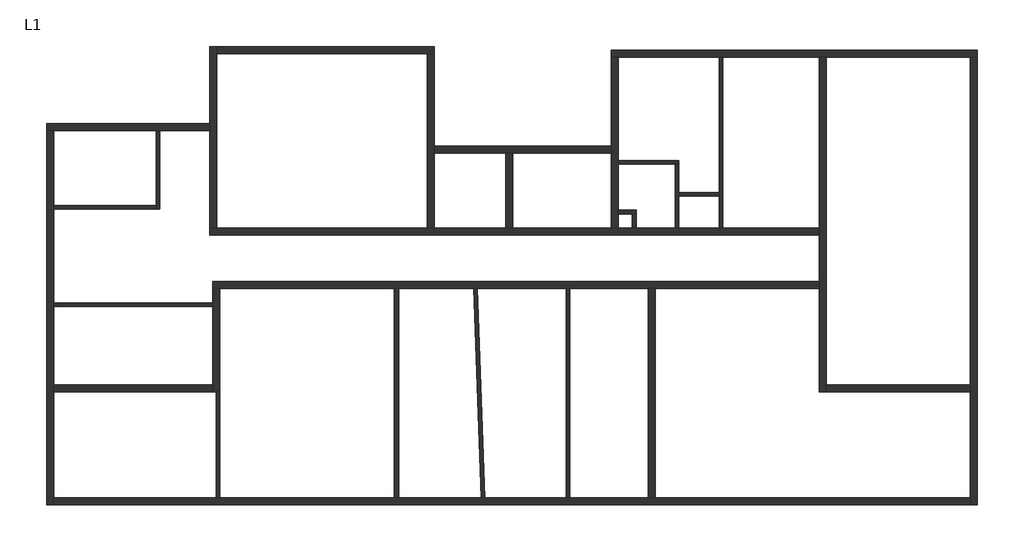
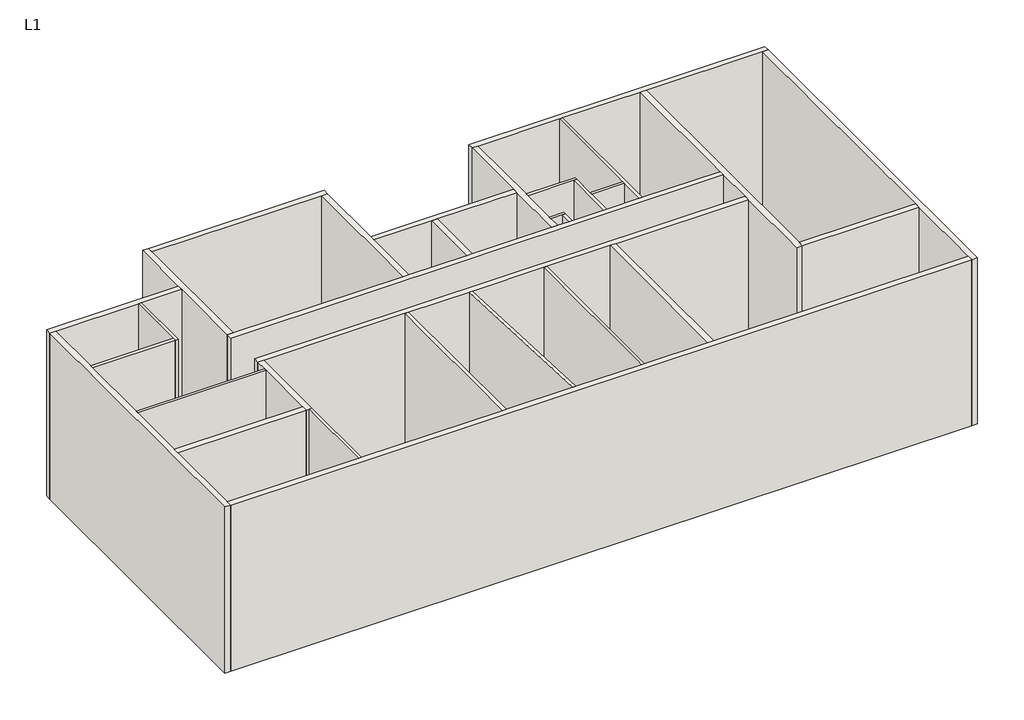
# One storey: 31 walls.
"""IFC4 building model written with IfcOpenShell, lengths in millimetres."""

from ifc_helpers import new_model, si_unit, origin, origin_with_axes, place, context, project, spatial, polyline, outline, extrude, faceted_brep, element, save

model = new_model("IFC4")

# Units and contexts
model_context = context("Model", 3, world=origin())
ifc_project = project(units=[si_unit("LENGTHUNIT", "METRE", prefix="MILLI")], contexts=[model_context])

# Site, building, storey
site = spatial("IfcSite", under=ifc_project)
building = spatial("IfcBuilding", under=site)
storey = spatial("IfcBuildingStorey", under=building, Name="L1", Elevation=0.0)

# Walls
placement = place(None, origin())
element("IfcWall", 1, ObjectType="Generic - 100mm", at=placement, inside=storey, context=model_context, shape_type="Brep", body=[
    faceted_brep([(-11422.4352558, 5591.031319, 0.0), (-11422.4352558, 3491.031319, 0.0), (-11422.4352558, 3391.031319, 0.0), (-11422.4352558, 3391.031319, 6096.0), (-11422.4352558, 3491.031319, 6096.0), (-11422.4352558, 5591.031319, 6096.0), (-11322.4352558, 5591.031319, 0.0), (-11322.4352558, 5591.031319, 6096.0), (-11322.4352558, 3391.031319, 6096.0), (-11322.4352558, 3391.031319, 0.0)], [[[0, 1, 2, 3, 4, 5]], [[6, 7, 8, 9]], [[2, 1, 0, 6, 9]], [[5, 4, 3, 8, 7]], [[0, 5, 7, 6]], [[3, 2, 9, 8]]]),
])
element("IfcWall", 2, ObjectType="Generic - 100mm", at=placement, inside=storey, context=model_context, shape_type="SweptSolid", body=[
    extrude(outline(polyline([(-14299.9378813, 3491.031319), (-11422.4352558, 3491.031319), (-11422.4352558, 3391.031319), (-14299.9378813, 3391.031319), (-14299.9378813, 3491.031319)])), origin_with_axes(), (0.0, 0.0, 1.0), 6096.0),
])
element("IfcWall", 3, ObjectType="Generic - 100mm", at=placement, inside=storey, context=model_context, shape_type="SweptSolid", body=[
    extrude(outline(polyline([(-9843.4352558, 651.031319), (-14299.9378813, 651.031319), (-14299.9378813, 751.031319), (-9843.4352558, 751.031319), (-9843.4352558, 651.031319)])), origin_with_axes(), (0.0, 0.0, 1.0), 6096.0),
])
element("IfcWall", 4, ObjectType="Generic - 100mm", at=placement, inside=storey, context=model_context, shape_type="SweptSolid", body=[
    extrude(outline(polyline([(-9643.4352558, -1748.968681), (-9643.4352558, -4724.7581907), (-9743.4352558, -4724.7581907), (-9743.4352558, -1748.968681), (-9643.4352558, -1748.968681)])), origin_with_axes(), (0.0, 0.0, 1.0), 6096.0),
])
element("IfcWall", 5, ObjectType="Generic - 100mm", at=placement, inside=storey, context=model_context, shape_type="SweptSolid", body=[
    extrude(outline(polyline([(-2303.3408114, -4724.7581907), (-2508.5279024, 1151.031319), (-2408.466948, 1151.031319), (-2203.2798569, -4724.7581907), (-2303.3408114, -4724.7581907)])), origin_with_axes(), (0.0, 0.0, 1.0), 6096.0),
])
element("IfcWall", 6, ObjectType="Generic - 100mm", at=placement, inside=storey, context=model_context, shape_type="SweptSolid", body=[
    extrude(outline(polyline([(77.5647442, -4724.7581907), (77.5647442, 1151.031319), (177.5647442, 1151.031319), (177.5647442, -4724.7581907), (77.5647442, -4724.7581907)])), origin_with_axes(), (0.0, 0.0, 1.0), 6096.0),
])
element("IfcWall", 7, ObjectType="Generic - 100mm", at=placement, inside=storey, context=model_context, shape_type="Brep", body=[
    faceted_brep([(4377.5647442, 7651.031319, 0.0), (4377.5647442, 3851.031319, 0.0), (4377.5647442, 3751.031319, 0.0), (4377.5647442, 2851.031319, 0.0), (4377.5647442, 2851.031319, 6096.0), (4377.5647442, 3751.031319, 6096.0), (4377.5647442, 3851.031319, 6096.0), (4377.5647442, 7651.031319, 6096.0), (4477.5647442, 7651.031319, 0.0), (4477.5647442, 7651.031319, 6096.0), (4477.5647442, 2851.031319, 6096.0), (4477.5647442, 2851.031319, 0.0)], [[[0, 1, 2, 3, 4, 5, 6, 7]], [[8, 9, 10, 11]], [[3, 2, 1, 0, 8, 11]], [[7, 6, 5, 4, 10, 9]], [[0, 7, 9, 8]], [[4, 3, 11, 10]]]),
])
element("IfcWall", 8, ObjectType="Generic - 100mm", at=placement, inside=storey, context=model_context, shape_type="Brep", body=[
    faceted_brep([(1538.9703153, 4651.031319, 0.0), (3138.9703153, 4651.031319, 0.0), (3238.9703153, 4651.031319, 0.0), (3238.9703153, 4651.031319, 6096.0), (3138.9703153, 4651.031319, 6096.0), (1538.9703153, 4651.031319, 6096.0), (1538.9703153, 4751.031319, 0.0), (1538.9703153, 4751.031319, 6096.0), (3238.9703153, 4751.031319, 6096.0), (3238.9703153, 4751.031319, 0.0)], [[[0, 1, 2, 3, 4, 5]], [[6, 7, 8, 9]], [[2, 1, 0, 6, 9]], [[5, 4, 3, 8, 7]], [[0, 5, 7, 6]], [[3, 2, 9, 8]]]),
])
element("IfcWall", 9, ObjectType="Generic - 100mm", at=placement, inside=storey, context=model_context, shape_type="Brep", body=[
    faceted_brep([(3138.9703153, 4651.031319, 0.0), (3138.9703153, 2851.031319, 0.0), (3138.9703153, 2851.031319, 6096.0), (3138.9703153, 4651.031319, 6096.0), (3238.9703153, 4651.031319, 0.0), (3238.9703153, 4651.031319, 6096.0), (3238.9703153, 3851.031319, 6096.0), (3238.9703153, 3751.031319, 6096.0), (3238.9703153, 2851.031319, 6096.0), (3238.9703153, 2851.031319, 0.0), (3238.9703153, 3751.031319, 0.0), (3238.9703153, 3851.031319, 0.0)], [[[0, 1, 2, 3]], [[4, 5, 6, 7, 8, 9, 10, 11]], [[1, 0, 4, 11, 10, 9]], [[3, 2, 8, 7, 6, 5]], [[0, 3, 5, 4]], [[2, 1, 9, 8]]]),
])
element("IfcWall", 10, ObjectType="Generic - 100mm", at=placement, inside=storey, context=model_context, shape_type="Brep", body=[
    faceted_brep([(1538.9703153, 3251.031319, 0.0), (1938.9703153, 3251.031319, 0.0), (2038.9703153, 3251.031319, 0.0), (2038.9703153, 3251.031319, 6096.0), (1938.9703153, 3251.031319, 6096.0), (1538.9703153, 3251.031319, 6096.0), (1538.9703153, 3351.031319, 0.0), (1538.9703153, 3351.031319, 6096.0), (2038.9703153, 3351.031319, 6096.0), (2038.9703153, 3351.031319, 0.0)], [[[0, 1, 2, 3, 4, 5]], [[6, 7, 8, 9]], [[2, 1, 0, 6, 9]], [[5, 4, 3, 8, 7]], [[0, 5, 7, 6]], [[3, 2, 9, 8]]]),
])
element("IfcWall", 11, ObjectType="Generic - 100mm", at=placement, inside=storey, context=model_context, shape_type="SweptSolid", body=[
    extrude(outline(polyline([(1938.9703153, 2851.031319), (1938.9703153, 3251.031319), (2038.9703153, 3251.031319), (2038.9703153, 2851.031319), (1938.9703153, 2851.031319)])), origin_with_axes(), (0.0, 0.0, 1.0), 6096.0),
])
element("IfcWall", 12, ObjectType="Generic - 100mm", at=placement, inside=storey, context=model_context, shape_type="SweptSolid", body=[
    extrude(outline(polyline([(4377.5647442, 3751.031319), (3238.9703153, 3751.031319), (3238.9703153, 3851.031319), (4377.5647442, 3851.031319), (4377.5647442, 3751.031319)])), origin_with_axes(), (0.0, 0.0, 1.0), 6096.0),
])
element("IfcWall", 13, ObjectType="Generic - 200mm", at=placement, inside=storey, context=model_context, shape_type="Brep", body=[
    faceted_brep([(11419.092187, 7651.031319, 0.0), (11419.092187, -1548.968681, 0.0), (11419.092187, -1748.968681, 0.0), (11419.092187, -4724.7581907, 0.0), (11419.092187, -4924.7581907, 0.0), (11419.092187, -4924.7581907, 6096.0), (11419.092187, -4724.7581907, 6096.0), (11419.092187, -1748.968681, 6096.0), (11419.092187, -1548.968681, 6096.0), (11419.092187, 7651.031319, 6096.0), (11619.092187, 7651.031319, 0.0), (11619.092187, 7651.031319, 6096.0), (11619.092187, -4924.7581907, 6096.0), (11619.092187, -4924.7581907, 0.0)], [[[0, 1, 2, 3, 4, 5, 6, 7, 8, 9]], [[10, 11, 12, 13]], [[4, 3, 2, 1, 0, 10, 13]], [[9, 8, 7, 6, 5, 12, 11]], [[5, 4, 13, 12]], [[0, 9, 11, 10]]]),
])
element("IfcWall", 14, ObjectType="Generic - 200mm", at=placement, inside=storey, context=model_context, shape_type="Brep", body=[
    faceted_brep([(11419.092187, -4724.7581907, 0.0), (2577.5647442, -4724.7581907, 0.0), (2377.5647442, -4724.7581907, 0.0), (177.5647442, -4724.7581907, 0.0), (77.5647442, -4724.7581907, 0.0), (-2203.2798569, -4724.7581907, 0.0), (-2303.3408114, -4724.7581907, 0.0), (-4622.4352558, -4724.7581907, 0.0), (-4743.4352558, -4724.7581907, 0.0), (-9643.4352558, -4724.7581907, 0.0), (-9743.4352558, -4724.7581907, 0.0), (-14299.9378813, -4724.7581907, 0.0), (-14299.9378813, -4724.7581907, 6096.0), (-9743.4352558, -4724.7581907, 6096.0), (-9643.4352558, -4724.7581907, 6096.0), (-4743.4352558, -4724.7581907, 6096.0), (-4622.4352558, -4724.7581907, 6096.0), (-2303.3408114, -4724.7581907, 6096.0), (-2203.2798569, -4724.7581907, 6096.0), (77.5647442, -4724.7581907, 6096.0), (177.5647442, -4724.7581907, 6096.0), (2377.5647442, -4724.7581907, 6096.0), (2577.5647442, -4724.7581907, 6096.0), (11419.092187, -4724.7581907, 6096.0), (11419.092187, -4924.7581907, 0.0), (11419.092187, -4924.7581907, 6096.0), (-14299.9378813, -4924.7581907, 6096.0), (-14299.9378813, -4924.7581907, 0.0)], [[[0, 1, 2, 3, 4, 5, 6, 7, 8, 9, 10, 11, 12, 13, 14, 15, 16, 17, 18, 19, 20, 21, 22, 23]], [[24, 25, 26, 27]], [[11, 10, 9, 8, 7, 6, 5, 4, 3, 2, 1, 0, 24, 27]], [[23, 22, 21, 20, 19, 18, 17, 16, 15, 14, 13, 12, 26, 25]], [[0, 23, 25, 24]], [[12, 11, 27, 26]]]),
])
element("IfcWall", 15, ObjectType="Generic - 200mm", at=placement, inside=storey, context=model_context, shape_type="Brep", body=[
    faceted_brep([(-14299.9378813, -4924.7581907, 0.0), (-14299.9378813, -4724.7581907, 0.0), (-14299.9378813, -1748.968681, 0.0), (-14299.9378813, -1548.968681, 0.0), (-14299.9378813, 651.031319, 0.0), (-14299.9378813, 751.031319, 0.0), (-14299.9378813, 3391.031319, 0.0), (-14299.9378813, 3491.031319, 0.0), (-14299.9378813, 5591.031319, 0.0), (-14299.9378813, 5591.031319, 6096.0), (-14299.9378813, 3491.031319, 6096.0), (-14299.9378813, 3391.031319, 6096.0), (-14299.9378813, 751.031319, 6096.0), (-14299.9378813, 651.031319, 6096.0), (-14299.9378813, -1548.968681, 6096.0), (-14299.9378813, -1748.968681, 6096.0), (-14299.9378813, -4724.7581907, 6096.0), (-14299.9378813, -4924.7581907, 6096.0), (-14499.9378813, -4924.7581907, 0.0), (-14499.9378813, -4924.7581907, 6096.0), (-14499.9378813, 5591.031319, 6096.0), (-14499.9378813, 5591.031319, 0.0)], [[[0, 1, 2, 3, 4, 5, 6, 7, 8, 9, 10, 11, 12, 13, 14, 15, 16, 17]], [[18, 19, 20, 21]], [[8, 7, 6, 5, 4, 3, 2, 1, 0, 18, 21]], [[17, 16, 15, 14, 13, 12, 11, 10, 9, 20, 19]], [[9, 8, 21, 20]], [[0, 17, 19, 18]]]),
])
element("IfcWall", 16, ObjectType="Generic - 200mm", at=placement, inside=storey, context=model_context, shape_type="Brep", body=[
    faceted_brep([(-14499.9378813, 5591.031319, 0.0), (-14299.9378813, 5591.031319, 0.0), (-11422.4352558, 5591.031319, 0.0), (-11322.4352558, 5591.031319, 0.0), (-9922.4352558, 5591.031319, 0.0), (-9922.4352558, 5591.031319, 6096.0), (-11322.4352558, 5591.031319, 6096.0), (-11422.4352558, 5591.031319, 6096.0), (-14299.9378813, 5591.031319, 6096.0), (-14499.9378813, 5591.031319, 6096.0), (-14499.9378813, 5791.031319, 0.0), (-14499.9378813, 5791.031319, 6096.0), (-9922.4352558, 5791.031319, 6096.0), (-9922.4352558, 5791.031319, 0.0)], [[[0, 1, 2, 3, 4, 5, 6, 7, 8, 9]], [[10, 11, 12, 13]], [[4, 3, 2, 1, 0, 10, 13]], [[9, 8, 7, 6, 5, 12, 11]], [[5, 4, 13, 12]], [[0, 9, 11, 10]]]),
])
element("IfcWall", 17, ObjectType="Generic - 200mm", at=placement, inside=storey, context=model_context, shape_type="Brep", body=[
    faceted_brep([(-9722.4352558, 2851.031319, 0.0), (-9722.4352558, 7751.031319, 0.0), (-9722.4352558, 7951.031319, 0.0), (-9722.4352558, 7951.031319, 6096.0), (-9722.4352558, 7751.031319, 6096.0), (-9722.4352558, 2851.031319, 6096.0), (-9922.4352558, 2851.031319, 0.0), (-9922.4352558, 2851.031319, 6096.0), (-9922.4352558, 5591.031319, 6096.0), (-9922.4352558, 5791.031319, 6096.0), (-9922.4352558, 7951.031319, 6096.0), (-9922.4352558, 7951.031319, 0.0), (-9922.4352558, 5791.031319, 0.0), (-9922.4352558, 5591.031319, 0.0)], [[[0, 1, 2, 3, 4, 5]], [[6, 7, 8, 9, 10, 11, 12, 13]], [[2, 1, 0, 6, 13, 12, 11]], [[5, 4, 3, 10, 9, 8, 7]], [[3, 2, 11, 10]], [[0, 5, 7, 6]]]),
])
element("IfcWall", 18, ObjectType="Generic - 200mm", at=placement, inside=storey, context=model_context, shape_type="Brep", body=[
    faceted_brep([(-9722.4352558, 7751.031319, 0.0), (-3822.4352558, 7751.031319, 0.0), (-3622.4352558, 7751.031319, 0.0), (-3622.4352558, 7751.031319, 6096.0), (-3822.4352558, 7751.031319, 6096.0), (-9722.4352558, 7751.031319, 6096.0), (-9722.4352558, 7951.031319, 0.0), (-9722.4352558, 7951.031319, 6096.0), (-3622.4352558, 7951.031319, 6096.0), (-3622.4352558, 7951.031319, 0.0)], [[[0, 1, 2, 3, 4, 5]], [[6, 7, 8, 9]], [[2, 1, 0, 6, 9]], [[5, 4, 3, 8, 7]], [[0, 5, 7, 6]], [[3, 2, 9, 8]]]),
])
element("IfcWall", 19, ObjectType="Generic - 200mm", at=placement, inside=storey, context=model_context, shape_type="Brep", body=[
    faceted_brep([(-3822.4352558, 7751.031319, 0.0), (-3822.4352558, 2851.031319, 0.0), (-3822.4352558, 2851.031319, 6096.0), (-3822.4352558, 7751.031319, 6096.0), (-3622.4352558, 7751.031319, 0.0), (-3622.4352558, 7751.031319, 6096.0), (-3622.4352558, 5151.031319, 6096.0), (-3622.4352558, 4951.031319, 6096.0), (-3622.4352558, 2851.031319, 6096.0), (-3622.4352558, 2851.031319, 0.0), (-3622.4352558, 4951.031319, 0.0), (-3622.4352558, 5151.031319, 0.0)], [[[0, 1, 2, 3]], [[4, 5, 6, 7, 8, 9, 10, 11]], [[1, 0, 4, 11, 10, 9]], [[3, 2, 8, 7, 6, 5]], [[0, 3, 5, 4]], [[2, 1, 9, 8]]]),
])
element("IfcWall", 20, ObjectType="Generic - 200mm", at=placement, inside=storey, context=model_context, shape_type="Brep", body=[
    faceted_brep([(-3622.4352558, 4951.031319, 0.0), (-1622.4352558, 4951.031319, 0.0), (-1422.4352558, 4951.031319, 0.0), (1338.9703153, 4951.031319, 0.0), (1338.9703153, 4951.031319, 6096.0), (-1422.4352558, 4951.031319, 6096.0), (-1622.4352558, 4951.031319, 6096.0), (-3622.4352558, 4951.031319, 6096.0), (-3622.4352558, 5151.031319, 0.0), (-3622.4352558, 5151.031319, 6096.0), (1338.9703153, 5151.031319, 6096.0), (1338.9703153, 5151.031319, 0.0)], [[[0, 1, 2, 3, 4, 5, 6, 7]], [[8, 9, 10, 11]], [[3, 2, 1, 0, 8, 11]], [[7, 6, 5, 4, 10, 9]], [[0, 7, 9, 8]], [[4, 3, 11, 10]]]),
])
element("IfcWall", 21, ObjectType="Generic - 200mm", at=placement, inside=storey, context=model_context, shape_type="Brep", body=[
    faceted_brep([(1338.9703153, 7651.031319, 0.0), (1538.9703153, 7651.031319, 0.0), (4377.5647442, 7651.031319, 0.0), (4477.5647442, 7651.031319, 0.0), (7177.5647442, 7651.031319, 0.0), (7377.5647442, 7651.031319, 0.0), (11419.092187, 7651.031319, 0.0), (11619.092187, 7651.031319, 0.0), (11619.092187, 7651.031319, 6096.0), (11419.092187, 7651.031319, 6096.0), (7377.5647442, 7651.031319, 6096.0), (7177.5647442, 7651.031319, 6096.0), (4477.5647442, 7651.031319, 6096.0), (4377.5647442, 7651.031319, 6096.0), (1538.9703153, 7651.031319, 6096.0), (1338.9703153, 7651.031319, 6096.0), (1338.9703153, 7851.031319, 0.0), (1338.9703153, 7851.031319, 6096.0), (11619.092187, 7851.031319, 6096.0), (11619.092187, 7851.031319, 0.0)], [[[0, 1, 2, 3, 4, 5, 6, 7, 8, 9, 10, 11, 12, 13, 14, 15]], [[16, 17, 18, 19]], [[7, 6, 5, 4, 3, 2, 1, 0, 16, 19]], [[15, 14, 13, 12, 11, 10, 9, 8, 18, 17]], [[8, 7, 19, 18]], [[0, 15, 17, 16]]]),
])
element("IfcWall", 22, ObjectType="Generic - 200mm", at=placement, inside=storey, context=model_context, shape_type="Brep", body=[
    faceted_brep([(7177.5647442, 7651.031319, 0.0), (7177.5647442, 2851.031319, 0.0), (7177.5647442, 2651.031319, 0.0), (7177.5647442, 1351.031319, 0.0), (7177.5647442, 1151.031319, 0.0), (7177.5647442, -1748.968681, 0.0), (7177.5647442, -1748.968681, 6096.0), (7177.5647442, 1151.031319, 6096.0), (7177.5647442, 1351.031319, 6096.0), (7177.5647442, 2651.031319, 6096.0), (7177.5647442, 2851.031319, 6096.0), (7177.5647442, 7651.031319, 6096.0), (7377.5647442, 7651.031319, 0.0), (7377.5647442, 7651.031319, 6096.0), (7377.5647442, -1548.968681, 6096.0), (7377.5647442, -1748.968681, 6096.0), (7377.5647442, -1748.968681, 0.0), (7377.5647442, -1548.968681, 0.0)], [[[0, 1, 2, 3, 4, 5, 6, 7, 8, 9, 10, 11]], [[12, 13, 14, 15, 16, 17]], [[5, 4, 3, 2, 1, 0, 12, 17, 16]], [[11, 10, 9, 8, 7, 6, 15, 14, 13]], [[0, 11, 13, 12]], [[6, 5, 16, 15]]]),
])
element("IfcWall", 23, ObjectType="Generic - 200mm", at=placement, inside=storey, context=model_context, shape_type="Brep", body=[
    faceted_brep([(7177.5647442, 2851.031319, 0.0), (4477.5647442, 2851.031319, 0.0), (4377.5647442, 2851.031319, 0.0), (3238.9703153, 2851.031319, 0.0), (3138.9703153, 2851.031319, 0.0), (2038.9703153, 2851.031319, 0.0), (1938.9703153, 2851.031319, 0.0), (1538.9703153, 2851.031319, 0.0), (1338.9703153, 2851.031319, 0.0), (-1422.4352558, 2851.031319, 0.0), (-1622.4352558, 2851.031319, 0.0), (-3622.4352558, 2851.031319, 0.0), (-3822.4352558, 2851.031319, 0.0), (-9722.4352558, 2851.031319, 0.0), (-9922.4352558, 2851.031319, 0.0), (-9922.4352558, 2851.031319, 6096.0), (-9722.4352558, 2851.031319, 6096.0), (-3822.4352558, 2851.031319, 6096.0), (-3622.4352558, 2851.031319, 6096.0), (-1622.4352558, 2851.031319, 6096.0), (-1422.4352558, 2851.031319, 6096.0), (1338.9703153, 2851.031319, 6096.0), (1538.9703153, 2851.031319, 6096.0), (1938.9703153, 2851.031319, 6096.0), (2038.9703153, 2851.031319, 6096.0), (3138.9703153, 2851.031319, 6096.0), (3238.9703153, 2851.031319, 6096.0), (4377.5647442, 2851.031319, 6096.0), (4477.5647442, 2851.031319, 6096.0), (7177.5647442, 2851.031319, 6096.0), (7177.5647442, 2651.031319, 0.0), (7177.5647442, 2651.031319, 6096.0), (-9922.4352558, 2651.031319, 6096.0), (-9922.4352558, 2651.031319, 0.0)], [[[0, 1, 2, 3, 4, 5, 6, 7, 8, 9, 10, 11, 12, 13, 14, 15, 16, 17, 18, 19, 20, 21, 22, 23, 24, 25, 26, 27, 28, 29]], [[30, 31, 32, 33]], [[14, 13, 12, 11, 10, 9, 8, 7, 6, 5, 4, 3, 2, 1, 0, 30, 33]], [[29, 28, 27, 26, 25, 24, 23, 22, 21, 20, 19, 18, 17, 16, 15, 32, 31]], [[0, 29, 31, 30]], [[15, 14, 33, 32]]]),
])
element("IfcWall", 24, ObjectType="Generic - 200mm", at=placement, inside=storey, context=model_context, shape_type="SweptSolid", body=[
    extrude(outline(polyline([(11419.092187, -1748.968681), (7377.5647442, -1748.968681), (7377.5647442, -1548.968681), (11419.092187, -1548.968681), (11419.092187, -1748.968681)])), origin_with_axes(), (0.0, 0.0, 1.0), 6096.0),
])
element("IfcWall", 25, ObjectType="Generic - 200mm", at=placement, inside=storey, context=model_context, shape_type="Brep", body=[
    faceted_brep([(7177.5647442, 1351.031319, 0.0), (-9843.4352558, 1351.031319, 0.0), (-9843.4352558, 1351.031319, 6096.0), (7177.5647442, 1351.031319, 6096.0), (7177.5647442, 1151.031319, 0.0), (7177.5647442, 1151.031319, 6096.0), (2577.5647442, 1151.031319, 6096.0), (2377.5647442, 1151.031319, 6096.0), (177.5647442, 1151.031319, 6096.0), (77.5647442, 1151.031319, 6096.0), (-2408.466948, 1151.031319, 6096.0), (-2508.5279024, 1151.031319, 6096.0), (-4622.4352558, 1151.031319, 6096.0), (-4743.4352558, 1151.031319, 6096.0), (-9643.4352558, 1151.031319, 6096.0), (-9843.4352558, 1151.031319, 6096.0), (-9843.4352558, 1151.031319, 0.0), (-9643.4352558, 1151.031319, 0.0), (-4743.4352558, 1151.031319, 0.0), (-4622.4352558, 1151.031319, 0.0), (-2508.5279024, 1151.031319, 0.0), (-2408.466948, 1151.031319, 0.0), (77.5647442, 1151.031319, 0.0), (177.5647442, 1151.031319, 0.0), (2377.5647442, 1151.031319, 0.0), (2577.5647442, 1151.031319, 0.0)], [[[0, 1, 2, 3]], [[4, 5, 6, 7, 8, 9, 10, 11, 12, 13, 14, 15, 16, 17, 18, 19, 20, 21, 22, 23, 24, 25]], [[1, 0, 4, 25, 24, 23, 22, 21, 20, 19, 18, 17, 16]], [[3, 2, 15, 14, 13, 12, 11, 10, 9, 8, 7, 6, 5]], [[0, 3, 5, 4]], [[2, 1, 16, 15]]]),
])
element("IfcWall", 26, ObjectType="Generic - 200mm", at=placement, inside=storey, context=model_context, shape_type="Brep", body=[
    faceted_brep([(-9843.4352558, 1151.031319, 0.0), (-9843.4352558, 751.031319, 0.0), (-9843.4352558, 651.031319, 0.0), (-9843.4352558, -1548.968681, 0.0), (-9843.4352558, -1748.968681, 0.0), (-9843.4352558, -1748.968681, 6096.0), (-9843.4352558, -1548.968681, 6096.0), (-9843.4352558, 651.031319, 6096.0), (-9843.4352558, 751.031319, 6096.0), (-9843.4352558, 1151.031319, 6096.0), (-9643.4352558, 1151.031319, 0.0), (-9643.4352558, 1151.031319, 6096.0), (-9643.4352558, -1748.968681, 6096.0), (-9643.4352558, -1748.968681, 0.0), (-9743.4352558, -1748.968681, 0.0), (-9743.4352558, -1748.968681, 6096.0)], [[[0, 1, 2, 3, 4, 5, 6, 7, 8, 9]], [[10, 11, 12, 13]], [[4, 3, 2, 1, 0, 10, 13, 14]], [[9, 8, 7, 6, 5, 15, 12, 11]], [[0, 9, 11, 10]], [[5, 4, 14, 13, 12, 15]]]),
])
element("IfcWall", 27, ObjectType="Generic - 200mm", at=placement, inside=storey, context=model_context, shape_type="SweptSolid", body=[
    extrude(outline(polyline([(-14299.9378813, -1548.968681), (-9843.4352558, -1548.968681), (-9843.4352558, -1748.968681), (-14299.9378813, -1748.968681), (-14299.9378813, -1548.968681)])), origin_with_axes(), (0.0, 0.0, 1.0), 6096.0),
])
element("IfcWall", 28, ObjectType="Generic - 200mm", at=placement, inside=storey, context=model_context, shape_type="SweptSolid", body=[
    extrude(outline(polyline([(2377.5647442, -4724.7581907), (2377.5647442, 1151.031319), (2577.5647442, 1151.031319), (2577.5647442, -4724.7581907), (2377.5647442, -4724.7581907)])), origin_with_axes(), (0.0, 0.0, 1.0), 6096.0),
])
element("IfcWall", 29, ObjectType="Generic - 200mm", at=placement, inside=storey, context=model_context, shape_type="SweptSolid", body=[
    extrude(outline(polyline([(-1622.4352558, 2851.031319), (-1622.4352558, 4951.031319), (-1422.4352558, 4951.031319), (-1422.4352558, 2851.031319), (-1622.4352558, 2851.031319)])), origin_with_axes(), (0.0, 0.0, 1.0), 6096.0),
])
element("IfcWall", 30, ObjectType="Generic - 200mm", at=placement, inside=storey, context=model_context, shape_type="Brep", body=[
    faceted_brep([(1338.9703153, 7651.031319, 0.0), (1338.9703153, 5151.031319, 0.0), (1338.9703153, 4951.031319, 0.0), (1338.9703153, 2851.031319, 0.0), (1338.9703153, 2851.031319, 6096.0), (1338.9703153, 4951.031319, 6096.0), (1338.9703153, 5151.031319, 6096.0), (1338.9703153, 7651.031319, 6096.0), (1538.9703153, 7651.031319, 0.0), (1538.9703153, 7651.031319, 6096.0), (1538.9703153, 4751.031319, 6096.0), (1538.9703153, 4651.031319, 6096.0), (1538.9703153, 3351.031319, 6096.0), (1538.9703153, 3251.031319, 6096.0), (1538.9703153, 2851.031319, 6096.0), (1538.9703153, 2851.031319, 0.0), (1538.9703153, 3251.031319, 0.0), (1538.9703153, 3351.031319, 0.0), (1538.9703153, 4651.031319, 0.0), (1538.9703153, 4751.031319, 0.0)], [[[0, 1, 2, 3, 4, 5, 6, 7]], [[8, 9, 10, 11, 12, 13, 14, 15, 16, 17, 18, 19]], [[3, 2, 1, 0, 8, 19, 18, 17, 16, 15]], [[7, 6, 5, 4, 14, 13, 12, 11, 10, 9]], [[4, 3, 15, 14]], [[0, 7, 9, 8]]]),
])
element("IfcWall", 31, ObjectType="Interior - 121mm Partition (1-hr)", at=placement, inside=storey, context=model_context, shape_type="SweptSolid", body=[
    extrude(outline(polyline([(-4743.4352558, -4724.7581907), (-4743.4352558, 1151.031319), (-4622.4352558, 1151.031319), (-4622.4352558, -4724.7581907), (-4743.4352558, -4724.7581907)])), origin_with_axes(), (0.0, 0.0, 1.0), 6096.0),
])

save(model, "model.ifc")

# Revit data of these elements
# Project information
#   Organization Name = "Organization Name"
#   Organization Description = "Organization Description"
#   Building Name = "Building Name"
#   Project Issue Date = "Issue Date"
#   Project Status = "Project Status"
#   Client Name = "Client Name"
#   Project Address = "Enter address here\nAddress Line 2"
#   Project Name = "Project Name"
#   Project Number = "Project Number"
# Type "Generic - 100mm"
#   Description = "Generic Wall (Material By Category), 100mm thick"
#   Assembly Code = "B2010"
#   Type Mark = "G01"
#   Layers, outside or top first: 100 mm no material (function 1)
# Type "Generic - 200mm"
#   Description = "Generic Wall (Material By Category), 200mm thick"
#   Assembly Code = "B2010"
#   Type Mark = "G06"
#   Layers, outside or top first: 200 mm no material (function 1)
# Type "Interior - 121mm Partition (1-hr)"
#   Description = "Wood Studs with one layer of Gypsum Wall Board (GWB) each side, Interior Function"
#   Assembly Code = "C1010145"
#   Type Mark = "P03"
#   Fire Rating = "1 HR"
#   Layers, outside or top first: 16 mm "Gypsum Wall Board" (function 5); 89 mm "Softwood, Lumber" (function 1); 16 mm "Gypsum Wall Board" (function 5)
# Elements 1, 2, 3, 4, 5, 6, 7, 8, 9, 10, 11, 12 (IfcWall, "Generic - 100mm")
#   Top Offset = 0 mm
#   Base Offset = 0 mm
#   Unconnected Height = 6096 mm
#   wall height = 6096 mm
#   Phase Created = New Construction
#   Base Constraint = L1
#   Materials on its faces: "Default Wall"
# Elements 13, 14, 15, 16, 17, 18, 19, 20, 21, 22, 23, 24, 25, 26, 27, 28, 29, 30 (IfcWall, "Generic - 200mm")
#   Top Offset = 0 mm
#   Base Offset = 0 mm
#   Unconnected Height = 6096 mm
#   wall height = 6096 mm
#   Phase Created = New Construction
#   Base Constraint = L1
#   Materials on its faces: "Default Wall"
# Element 31 (IfcWall, "Interior - 121mm Partition (1-hr)")
#   Top Offset = 0 mm
#   Base Offset = 0 mm
#   Unconnected Height = 6096 mm
#   wall height = 6096 mm
#   Phase Created = New Construction
#   Base Constraint = L1
#   Materials on its faces: "Default Wall", "Gypsum Wall Board"
# Materials
#   "Gypsum Wall Board": class "Generic", colour RGB 221 221 219, transparency 0, Description = "Gypsum Wall Board", Cost = 0
#   "Softwood, Lumber": class "Wood", colour RGB 230 189 133, transparency 0, Description = "Pinus Echinata", Cost = 0
#   "Default Wall": class "Miscellaneous", colour RGB 192 192 192, transparency 0, Cost = 0
